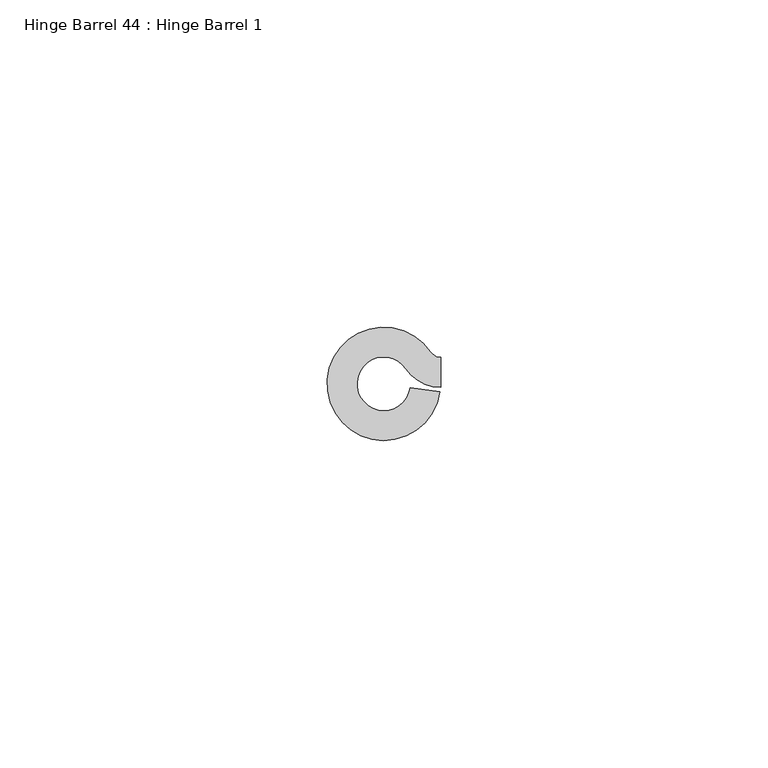
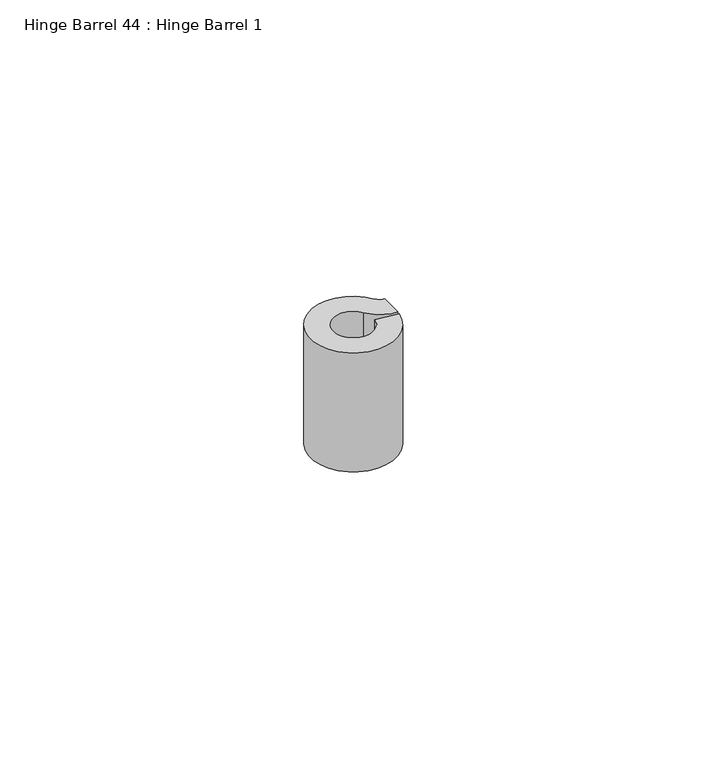
"""IFC4 building model written with IfcOpenShell, lengths in millimetres: proxy geometry, Hinge Barrel 44 : Hinge Barrel 1."""

from ifc_helpers import new_model, si_unit, point, frame, frame_2d, origin, place, context, project, spatial, polyline, circle_curve, trimmed, segment, composite_curve, outline, extrude, source, transform, mapped, element, save


def hinge_barrel_44_hinge_barrel_1_4b375d58(model_context):
    return source(origin(), model_context, "Body", "SweptSolid", [
        extrude(outline(composite_curve([segment(trimmed(circle_curve(frame_2d((587319.1320739, -534100.7049841)), 4.0894), [point((587322.5194669, -534098.4139665))], [point((587323.1821338, -534101.2708529))], True, "CARTESIAN"), True, "CONTINUOUS"), segment(polyline([(587323.1821338, -534101.2708529), (587327.7022899, -534101.9024028)]), True, "CONTINUOUS"), segment(trimmed(circle_curve(frame_2d((587319.1320739, -534100.7049841)), 8.6534625), [point((587327.7022899, -534101.9024028))], [point((587326.3000393, -534095.8570273))], False, "CARTESIAN"), True, "CONTINUOUS"), segment(trimmed(circle_curve(frame_2d((587327.8245257, -534094.8259615)), 1.8404226), [point((587326.3000393, -534095.8570273))], [point((587327.8245257, -534096.6663841))], True, "CARTESIAN"), True, "CONTINUOUS"), segment(polyline([(587327.8245257, -534096.6663841), (587327.8245257, -534101.2304466)]), True, "CONTINUOUS"), segment(trimmed(circle_curve(frame_2d((587327.8245257, -534094.8259615)), 6.4044851), [point((587327.8245257, -534101.2304466))], [point((587322.5194669, -534098.4139665))], False, "CARTESIAN"), True, "CONTINUOUS")], self_intersect=False)), frame((0.0, 0.0, 1962.15), z_axis=(0.0, 0.0, 1.0), x_axis=(1.0, 0.0, 0.0)), (0.0, 0.0, 1.0), 25.4),
    ])


if __name__ == "__main__":
    model = new_model("IFC4")
    model_context = context("Model", 3, world=origin())
    ifc_project = project(units=[si_unit("LENGTHUNIT", "METRE", prefix="MILLI")], contexts=[model_context])
    site = spatial("IfcSite", under=ifc_project)
    building = spatial("IfcBuilding", under=site)
    placement = place(None, origin())
    hinge_barrel_44_hinge_barrel_1_shape = hinge_barrel_44_hinge_barrel_1_4b375d58(model_context)
    element("IfcBuildingElementProxy", 1, Name="Hinge Barrel 44 : Hinge Barrel 1", ObjectType="Hinge Barrel 44 : Hinge Barrel 1", at=placement, inside=building, context=model_context, shape_type="MappedRepresentation", body=[
        mapped(hinge_barrel_44_hinge_barrel_1_shape, transform((0.0, 0.0, 0.0), x_axis=(1.0, 0.0, 0.0), y_axis=(0.0, 1.0, 0.0), z_axis=(0.0, 0.0, 1.0))),
    ])
    save(model, "model.ifc")

# Revit data of these elements
# Element 1 (IfcBuildingElementProxy, "Hinge Barrel 44 : Hinge Barrel 1")
#   Materials on its faces: "6\"X6\" WELD-ON STL BUTT HINGE"
# Materials
#   "6\"X6\" WELD-ON STL BUTT HINGE": class "Metal", colour RGB 189 187 185, transparency 0, Description = "Carbon steel", Cost = 0
